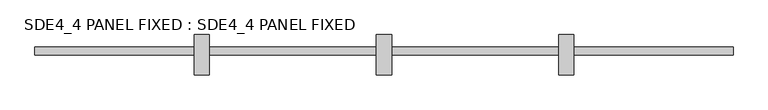
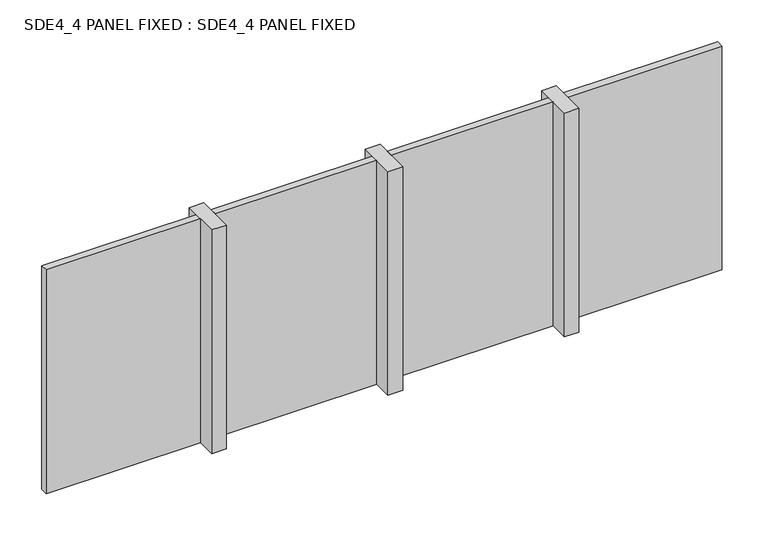
"""IFC4 building model written with IfcOpenShell, lengths in millimetres: plate geometry, SDE4_4 PANEL FIXED : SDE4_4 PANEL FIXED."""

from ifc_helpers import new_model, si_unit, origin, origin_with_axes, place, context, project, spatial, polyline, outline, extrude, source, transform, mapped, element, save


def sde4_4_panel_fixed_sde4_4_panel_fixed_ba0f1020(model_context):
    return source(origin(), model_context, "Body", "SweptSolid", [
        extrude(outline(polyline([(-1150.0, 132.5), (-1150.0, -132.5), (-1250.0, -132.5), (-1250.0, 132.5), (-1150.0, 132.5)])), origin_with_axes(), (0.0, 0.0, 1.0), 1610.4043686),
        extrude(outline(polyline([(50.0, 132.5), (50.0, -132.5), (-50.0, -132.5), (-50.0, 132.5), (50.0, 132.5)])), origin_with_axes(), (0.0, 0.0, 1.0), 1610.4043686),
        extrude(outline(polyline([(1250.0, 132.5), (1250.0, -132.5), (1150.0, -132.5), (1150.0, 132.5), (1250.0, 132.5)])), origin_with_axes(), (0.0, 0.0, 1.0), 1610.4043686),
        extrude(outline(polyline([(2299.0, 50.0), (2299.0, 0.0), (1250.0, 0.0), (1250.0, 50.0), (2299.0, 50.0)])), origin_with_axes(), (0.0, 0.0, 1.0), 1610.4043686),
        extrude(outline(polyline([(1150.0, 50.0), (1150.0, 0.0), (50.0, 0.0), (50.0, 50.0), (1150.0, 50.0)])), origin_with_axes(), (0.0, 0.0, 1.0), 1610.4043686),
        extrude(outline(polyline([(-50.0, 50.0), (-50.0, 0.0), (-1150.0, 0.0), (-1150.0, 50.0), (-50.0, 50.0)])), origin_with_axes(), (0.0, 0.0, 1.0), 1610.4043686),
        extrude(outline(polyline([(-1250.0, 50.0), (-1250.0, 0.0), (-2300.0, 0.0), (-2300.0, 50.0), (-1250.0, 50.0)])), origin_with_axes(), (0.0, 0.0, 1.0), 1610.4043686),
    ])


if __name__ == "__main__":
    model = new_model("IFC4")
    model_context = context("Model", 3, world=origin())
    ifc_project = project(units=[si_unit("LENGTHUNIT", "METRE", prefix="MILLI")], contexts=[model_context])
    site = spatial("IfcSite", under=ifc_project)
    building = spatial("IfcBuilding", under=site)
    placement = place(None, origin())
    sde4_4_panel_fixed_sde4_4_panel_fixed_shape = sde4_4_panel_fixed_sde4_4_panel_fixed_ba0f1020(model_context)
    element("IfcPlate", 1, ObjectType="SDE4_4 PANEL FIXED : SDE4_4 PANEL FIXED", at=placement, inside=building, context=model_context, shape_type="MappedRepresentation", body=[
        mapped(sde4_4_panel_fixed_sde4_4_panel_fixed_shape, transform((0.0, 0.0, 0.0), x_axis=(1.0, 0.0, 0.0), y_axis=(0.0, 1.0, 0.0), z_axis=(0.0, 0.0, 1.0))),
    ])
    save(model, "model.ifc")

# Revit data of these elements
# Type "SDE4_4 PANEL FIXED : SDE4_4 PANEL FIXED"
#   Type Mark = "CW-GLASS"
#   Analytic Construction = "<None>"
#   Glass = Glass
#   Frame = Aluminium
# Element 1 (IfcPlate, "SDE4_4 PANEL FIXED : SDE4_4 PANEL FIXED")
#   Materials on its faces: "Glass", "Aluminium"
# Materials
#   "Glass": class "Glass", colour RGB 0 128 192, transparency 0.9, Keynote = "L40", Cost = 0
#   "Aluminium": class "Unassigned", colour RGB 247 247 247, transparency 0, Cost = 0
